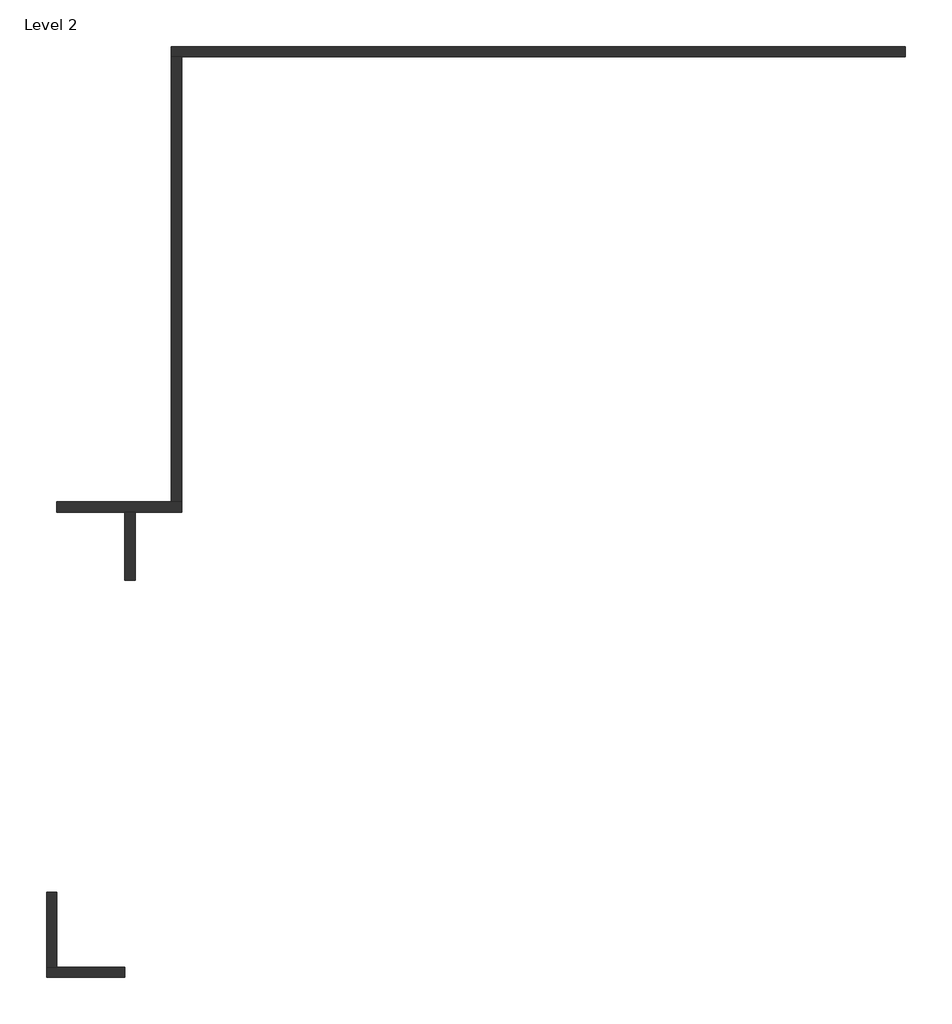
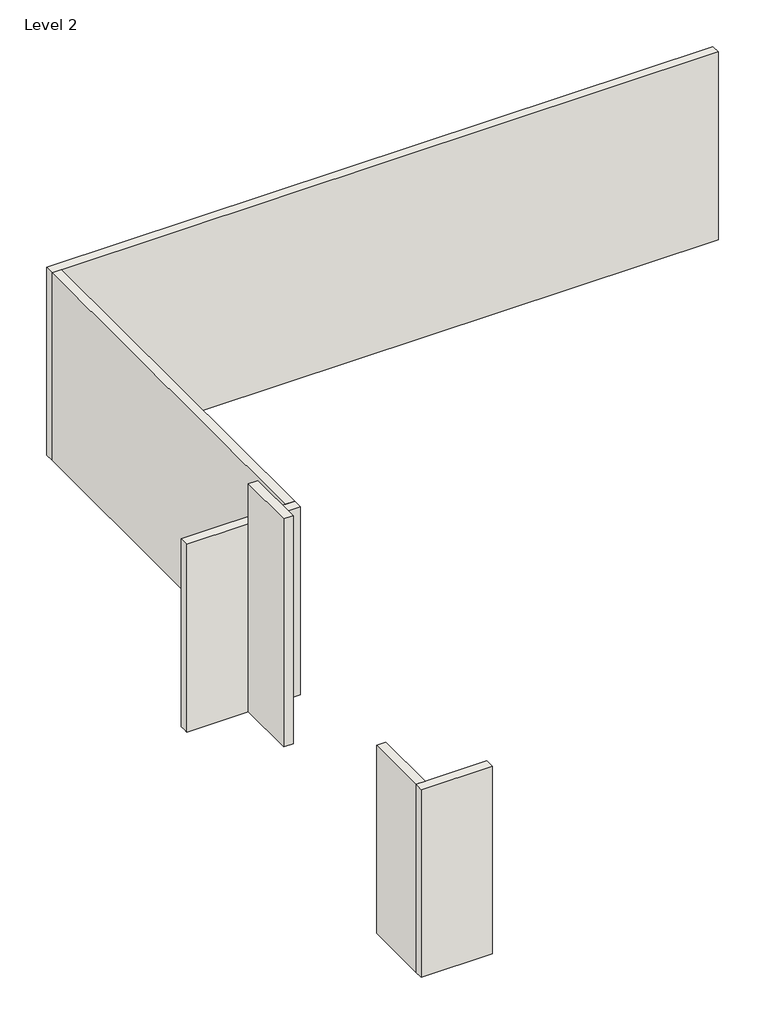
# One storey: 6 walls.
"""IFC4 building model written with IfcOpenShell, lengths in millimetres."""

from ifc_helpers import new_model, si_unit, frame, origin, place, context, project, spatial, polyline, outline, extrude, faceted_brep, element, save

model = new_model("IFC4")

# Units and contexts
model_context = context("Model", 3, world=origin())
ifc_project = project(units=[si_unit("LENGTHUNIT", "METRE", prefix="MILLI")], contexts=[model_context])

# Site, building, storey
site = spatial("IfcSite", under=ifc_project)
building = spatial("IfcBuilding", under=site)
storey = spatial("IfcBuildingStorey", under=building, Name="Level 2", Elevation=4876.8)

# Walls
placement = place(None, origin())
element("IfcWall", 1, ObjectType="Generic - 8\"", at=placement, inside=storey, context=model_context, shape_type="Brep", body=[
    faceted_brep([(18078.8737178, 8910.5120281, 4876.8), (3753.2737178, 8910.5120281, 4876.8), (3753.2737178, 8910.5120281, 9144.0), (18078.8737178, 8910.5120281, 9144.0), (18078.8737178, 8707.3120281, 4876.8), (18078.8737178, 8707.3120281, 9144.0), (3956.4737178, 8707.3120281, 9144.0), (3753.2737178, 8707.3120281, 9144.0), (3753.2737178, 8707.3120281, 4876.8), (3956.4737178, 8707.3120281, 4876.8)], [[[0, 1, 2, 3]], [[4, 5, 6, 7, 8, 9]], [[1, 0, 4, 9, 8]], [[3, 2, 7, 6, 5]], [[2, 1, 8, 7]], [[0, 3, 5, 4]]]),
])
element("IfcWall", 2, ObjectType="Generic - 8\"", at=placement, inside=storey, context=model_context, shape_type="Brep", body=[
    faceted_brep([(2838.8737178, -9058.4004719, 4876.8), (1518.0737178, -9058.4004719, 4876.8), (1314.8737178, -9058.4004719, 4876.8), (1314.8737178, -9058.4004719, 9144.0), (1518.0737178, -9058.4004719, 9144.0), (2838.8737178, -9058.4004719, 9144.0), (2838.8737178, -9058.4004719, 7315.2), (2838.8737178, -9261.6004719, 4876.8), (2838.8737178, -9261.6004719, 9144.0), (1314.8737178, -9261.6004719, 9144.0), (1314.8737178, -9261.6004719, 4876.8)], [[[0, 1, 2, 3, 4, 5, 6]], [[7, 8, 9, 10]], [[2, 1, 0, 7, 10]], [[5, 4, 3, 9, 8]], [[3, 2, 10, 9]], [[0, 6, 5, 8, 7]]]),
])
element("IfcWall", 3, ObjectType="Generic - 8\"", at=placement, inside=storey, context=model_context, shape_type="Brep", body=[
    faceted_brep([(1518.0737178, -9058.4004719, 4876.8), (1518.0737178, -7701.0879719, 4876.8), (1518.0737178, -7599.4879719, 4876.8), (1518.0737178, -7599.4879719, 9144.0), (1518.0737178, -9058.4004719, 9144.0), (1314.8737178, -9058.4004719, 4876.8), (1314.8737178, -9058.4004719, 9144.0), (1314.8737178, -7599.4879719, 9144.0), (1314.8737178, -7599.4879719, 4876.8), (1314.8737178, -7701.0879719, 4876.8)], [[[0, 1, 2, 3, 4]], [[5, 6, 7, 8, 9]], [[2, 1, 0, 5, 9, 8]], [[3, 2, 8, 7]], [[4, 3, 7, 6]], [[0, 4, 6, 5]]]),
])
element("IfcWall", 4, ObjectType="Generic - 8\"", at=placement, inside=storey, context=model_context, shape_type="SweptSolid", body=[
    extrude(outline(polyline([(3753.2737178, 20.5120281), (3753.2737178, 8707.3120281), (3956.4737178, 8707.3120281), (3956.4737178, 20.5120281), (3753.2737178, 20.5120281)])), frame((0.0, 0.0, 4876.8), z_axis=(0.0, 0.0, 1.0), x_axis=(1.0, 0.0, 0.0)), (0.0, 0.0, 1.0), 4267.2),
])
element("IfcWall", 5, ObjectType="Generic - 8\"", at=placement, inside=storey, context=model_context, shape_type="Brep", body=[
    faceted_brep([(3042.0737178, -1503.4879719, 4876.8), (3042.0737178, -182.6879719, 4876.8), (3042.0737178, -182.6879719, 10058.4), (3042.0737178, -1503.4879719, 10058.4), (3042.0737178, -1503.4879719, 9144.0), (2838.8737178, -1503.4879719, 4876.8), (2838.8737178, -1503.4879719, 9144.0), (2838.8737178, -1503.4879719, 10058.4), (2838.8737178, -182.6879719, 10058.4), (2838.8737178, -182.6879719, 4876.8)], [[[0, 1, 2, 3, 4]], [[5, 6, 7, 8, 9]], [[1, 0, 5, 9]], [[3, 2, 8, 7]], [[0, 4, 3, 7, 6, 5]], [[2, 1, 9, 8]]]),
])
element("IfcWall", 6, ObjectType="Generic - 8\"", at=placement, inside=storey, context=model_context, shape_type="Brep", body=[
    faceted_brep([(1518.0737178, -182.6879719, 4876.8), (2838.8737178, -182.6879719, 4876.8), (3042.0737178, -182.6879719, 4876.8), (3956.4737178, -182.6879719, 4876.8), (3956.4737178, -182.6879719, 9144.0), (1518.0737178, -182.6879719, 9144.0), (1518.0737178, 20.5120281, 4876.8), (1518.0737178, 20.5120281, 9144.0), (3753.2737178, 20.5120281, 9144.0), (3956.4737178, 20.5120281, 9144.0), (3956.4737178, 20.5120281, 4876.8), (3753.2737178, 20.5120281, 4876.8), (1518.0737178, -81.0879719, 4876.8)], [[[0, 1, 2, 3, 4, 5]], [[6, 7, 8, 9, 10, 11]], [[3, 2, 1, 0, 12, 6, 11, 10]], [[5, 4, 9, 8, 7]], [[0, 5, 7, 6, 12]], [[4, 3, 10, 9]]]),
])

save(model, "model.ifc")

# Revit data of these elements
# Project information
#   Project Issue Date = "Issue Date"
#   Project Status = "Project Status"
#   Client Name = "Owner"
#   Project Address = "Enter address here"
#   Project Name = "Project Name"
#   Project Number = "Project Number"
# Grids (mm)
#   "1": line (-18801.926, 15817.913) -> (-18801.926, -14896.109)
#   "2": line (-11486.726, 15817.913) -> (-11486.726, -14896.109)
#   "3": line (-4171.526, 15817.913) -> (-4171.526, -14896.109)
#   "4": line (3143.674, 15817.913) -> (3143.674, -14896.109)
#   "5": line (10458.874, 15817.913) -> (10458.874, -14896.109)
#   "6": line (17774.074, 15817.913) -> (17774.074, -14896.109)
#   "A": line (23913.763, 13177.712) -> (-22245.007, 13177.712)
#   "B": line (23913.763, 5862.512) -> (-22245.007, 5862.512)
#   "C": line (23913.763, -2671.888) -> (-22245.007, -2671.888)
#   "D": line (23913.763, -11206.288) -> (-22245.007, -11206.288)
# Type "Generic - 8\""
#   Assembly Code = "B2010"
#   Layers, outside or top first: 0' - 8" no material (function 1)
# Elements 1, 2, 3, 4, 6 (IfcWall, "Generic - 8\"")
#   Top Offset = 0' - 0"
#   Base Offset = 0' - 0"
#   wall height = 14' - 0"
#   Phase Created = New Construction
#   Base Constraint = Level 2
#   Top Constraint = Roof
#   Materials on its faces: "Default Wall"
# Element 5 (IfcWall, "Generic - 8\"")
#   Top Offset = 0' - 0"
#   Base Offset = 0' - 0"
#   wall height = 17' - 0"
#   Phase Created = New Construction
#   Base Constraint = Level 2
#   Top Constraint = Parapet
#   Materials on its faces: "Default Wall"
# Materials
#   "Default Wall": class "Miscellaneous", colour RGB 127 127 127, transparency 0, Cost = 0
